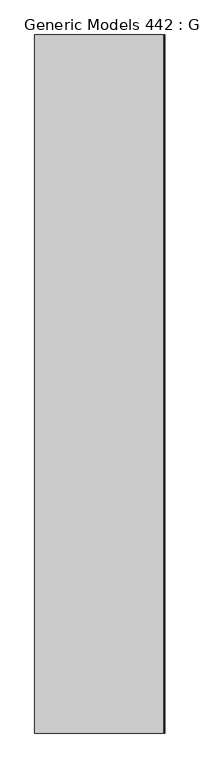
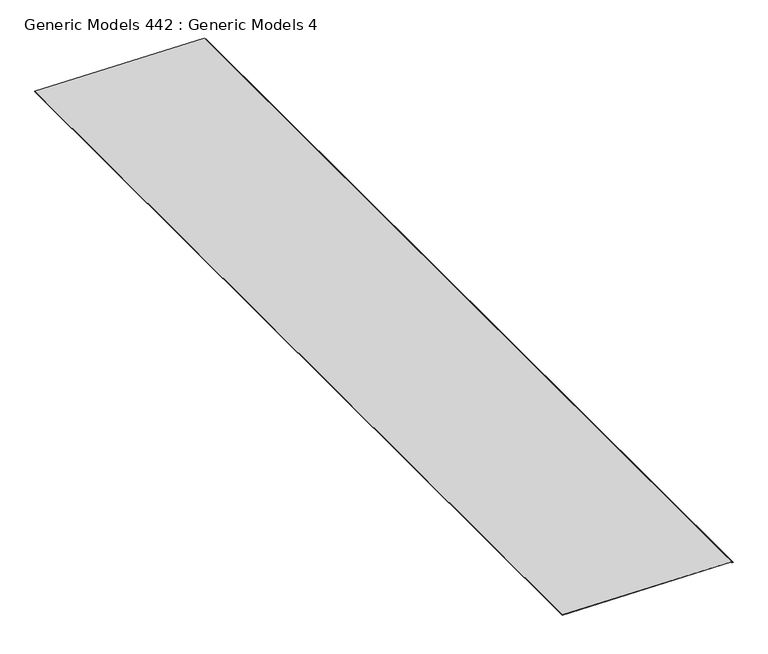
"""IFC4 building model written with IfcOpenShell, lengths in millimetres: proxy geometry, Generic Models 442 : Generic Models 4."""

from ifc_helpers import new_model, si_unit, frame, origin, place, context, project, spatial, polyline, outline, extrude, source, transform, mapped, element, save


def generic_models_442_generic_models_4_b700b8a6(model_context):
    return source(origin(), model_context, "Body", "SweptSolid", [
        extrude(outline(polyline([(126754.0315637, -8156.6058093), (126729.7082674, -6763.1250962), (126720.8812115, -6762.5078483), (126720.8812115, -6751.4950945), (126721.6749615, -6751.4950945), (126721.6749615, -6761.7676644), (126730.4892027, -6762.3840162), (126754.8251929, -8156.5919564), (126754.0315637, -8156.6058093)])), frame((0.0, -464.1230338, 0.0), z_axis=(0.0, 1.0, 0.0), x_axis=(0.0, 0.0, 1.0)), (0.0, 0.0, 1.0), 7518.4),
    ])


if __name__ == "__main__":
    model = new_model("IFC4")
    model_context = context("Model", 3, world=origin())
    ifc_project = project(units=[si_unit("LENGTHUNIT", "METRE", prefix="MILLI")], contexts=[model_context])
    site = spatial("IfcSite", under=ifc_project)
    building = spatial("IfcBuilding", under=site)
    placement = place(None, origin())
    generic_models_442_generic_models_4_shape = generic_models_442_generic_models_4_b700b8a6(model_context)
    element("IfcBuildingElementProxy", 1, Name="Generic Models 442 : Generic Models 4", ObjectType="Generic Models 442 : Generic Models 4", at=placement, inside=building, context=model_context, shape_type="MappedRepresentation", body=[
        mapped(generic_models_442_generic_models_4_shape, transform((0.0, 0.0, 0.0), x_axis=(1.0, 0.0, 0.0), y_axis=(0.0, 1.0, 0.0), z_axis=(0.0, 0.0, 1.0))),
    ])
    save(model, "model.ifc")

# Revit data of these elements
# Element 1 (IfcBuildingElementProxy, "Generic Models 442 : Generic Models 4")
#   Materials on its faces: "_HYDROSTOP LIQUID MEMBRANE - FOLLOW MANU. RECOMMENDED INSTALLATION DETAILS"
# Materials
#   "_HYDROSTOP LIQUID MEMBRANE - FOLLOW MANU. RECOMMENDED INSTALLATION DETAILS": class "Generic", colour RGB 156 184 169, transparency 0, Cost = 0
